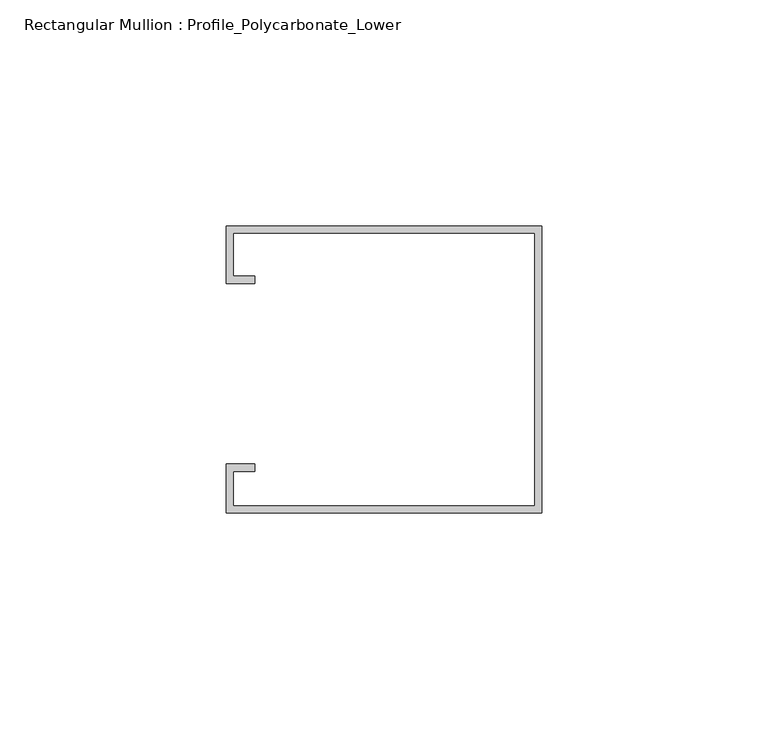
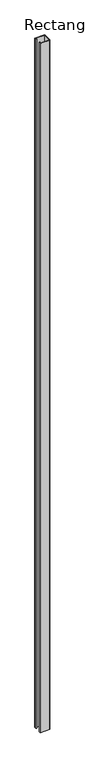
"""IFC4 building model written with IfcOpenShell, lengths in millimetres: member geometry, Rectangular Mullion : Profile_Polycarbonate_Lower."""

from ifc_helpers import new_model, si_unit, frame, origin, place, context, project, spatial, polyline, outline, extrude, source, transform, mapped, element, save


def rectangular_mullion_profile_polycarbonate_lower_bc9e4926(model_context):
    return source(origin(), model_context, "Body", "SweptSolid", [
        extrude(outline(polyline([(0.0, 32.7), (0.0, -30.8), (-69.85, -30.8), (-69.85, -20.0), (-63.5, -20.0), (-63.5, -21.5875), (-68.2625, -21.5875), (-68.2625, -29.2125), (-1.5875, -29.2125), (-1.5875, 31.1125), (-68.2625, 31.1125), (-68.2625, 21.5875), (-63.5, 21.5875), (-63.5, 20.0), (-69.85, 20.0), (-69.85, 32.7), (0.0, 32.7)])), frame((0.0, 0.0, -5180.0125), z_axis=(0.0, 0.0, 1.0), x_axis=(1.0, 0.0, 0.0)), (0.0, 0.0, 1.0), 5180.0125),
    ])


if __name__ == "__main__":
    model = new_model("IFC4")
    model_context = context("Model", 3, world=origin())
    ifc_project = project(units=[si_unit("LENGTHUNIT", "METRE", prefix="MILLI")], contexts=[model_context])
    site = spatial("IfcSite", under=ifc_project)
    building = spatial("IfcBuilding", under=site)
    placement = place(None, origin())
    rectangular_mullion_profile_polycarbonate_lower_shape = rectangular_mullion_profile_polycarbonate_lower_bc9e4926(model_context)
    element("IfcMember", 1, ObjectType="Rectangular Mullion : Profile_Polycarbonate_Lower", at=placement, inside=building, context=model_context, shape_type="MappedRepresentation", body=[
        mapped(rectangular_mullion_profile_polycarbonate_lower_shape, transform((0.0, 0.0, 0.0), x_axis=(1.0, 0.0, 0.0), y_axis=(0.0, 1.0, 0.0), z_axis=(0.0, 0.0, 1.0))),
    ])
    save(model, "model.ifc")

# Revit data of these elements
# Type "Rectangular Mullion : Profile_Polycarbonate_Lower"
#   built-in parameter 1007322 = 0.208333 (stored number, unit not read)
#   built-in parameter 1007321 = 0 (stored number, unit not read)
#   built-in parameter 1007320 = 0.00520833 (stored number, unit not read)
# Element 1 (IfcMember, "Rectangular Mullion : Profile_Polycarbonate_Lower")
#   Materials on its faces: "ALUMINUM PROFILE AT POLYCARBONATE PANEL"
# Materials
#   "ALUMINUM PROFILE AT POLYCARBONATE PANEL": class "Metal", colour RGB 244 244 244, transparency 0, Description = "Aluminum 6061", Cost = 0
